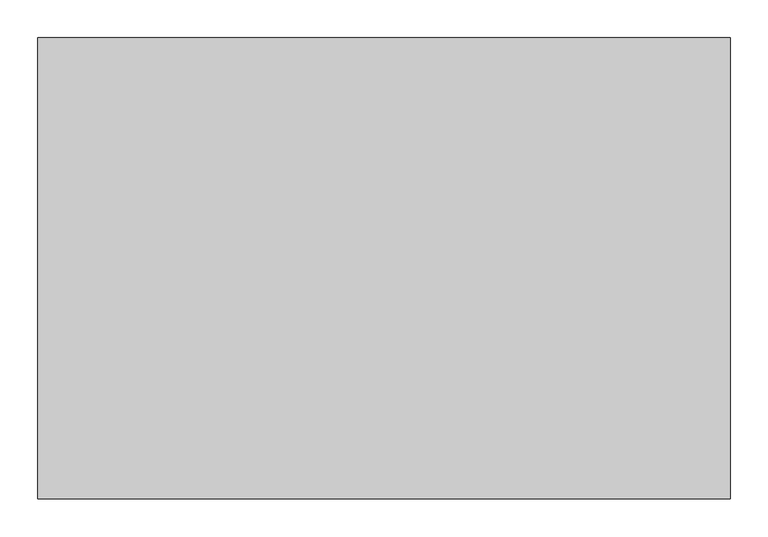
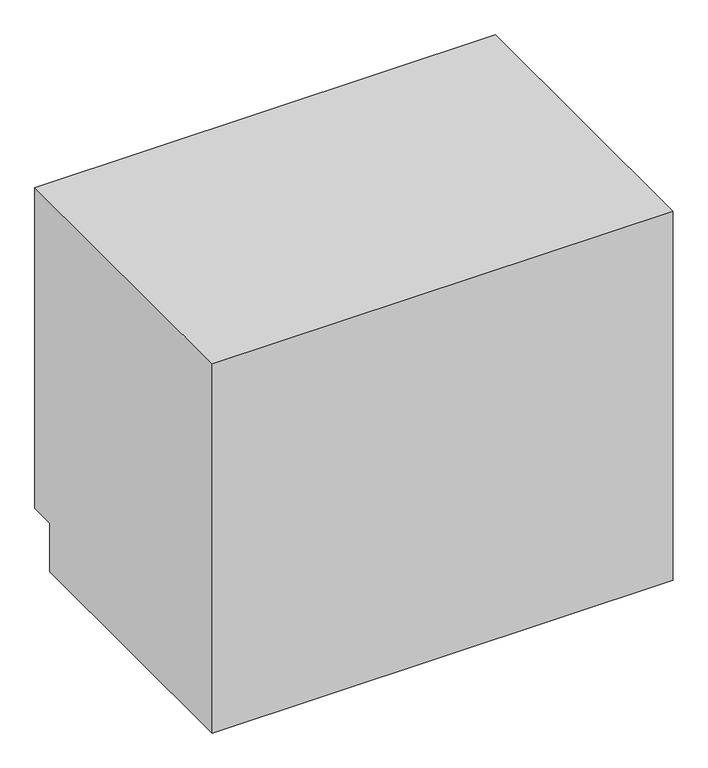
"""IFC4 building model written with IfcOpenShell, lengths in millimetres: furniture geometry, Cabinet, Base Doors and Drawers-NON-COLLECTUS : -."""

from ifc_helpers import new_model, si_unit, frame, origin, place, context, project, spatial, polyline, outline, extrude, source, transform, mapped, element, save


def furniture_34c6b9d5(model_context):
    return source(origin(), model_context, "Body", "SweptSolid", [
        extrude(outline(polyline([(-1384.3, 774.6984506), (-1384.3, 101.6), (-1435.1, 101.6), (-1435.1, 0.0), (-1993.8987808, 0.0), (-1993.8987808, 774.6984506), (-1384.3, 774.6984506)])), frame((114.3, 0.0, 0.0), z_axis=(1.0, 0.0, 0.0), x_axis=(0.0, 1.0, 0.0)), (0.0, 0.0, 1.0), 914.3981712),
    ])


if __name__ == "__main__":
    model = new_model("IFC4")
    model_context = context("Model", 3, world=origin())
    ifc_project = project(units=[si_unit("LENGTHUNIT", "METRE", prefix="MILLI")], contexts=[model_context])
    site = spatial("IfcSite", under=ifc_project)
    building = spatial("IfcBuilding", under=site)
    placement = place(None, origin())
    furniture_shape = furniture_34c6b9d5(model_context)
    element("IfcFurniture", 1, ObjectType="Cabinet, Base Doors and Drawers-NON-COLLECTUS : -", at=placement, inside=building, context=model_context, shape_type="MappedRepresentation", body=[
        mapped(furniture_shape, transform((0.0, 0.0, 0.0), x_axis=(1.0, 0.0, 0.0), y_axis=(0.0, 1.0, 0.0), z_axis=(0.0, 0.0, 1.0))),
    ])
    save(model, "model.ifc")

# Revit data of these elements
# Type "Cabinet, Base Doors and Drawers-NON-COLLECTUS : -"
#   External ID [instance default] = ""
#   Width Reporting [instance default] = 762 mm
#   Width [instance default] = 762 mm
#   Toe Kick Height = 101.6 mm
#   Toe Kick Depth = 50.8 mm
#   Height of Drawers = 152.4 mm
#   Height Reporting [instance default] = 825.5 mm
#   Height [instance default] = 825.5 mm
#   Depth Reporting [instance default] = 609.6 mm
#   Depth [instance default] = 609.6 mm
#   Material = White
#   Default Elevation = 0
# Element 1 (IfcFurniture, "Cabinet, Base Doors and Drawers-NON-COLLECTUS : -")
#   Width Reporting = 914.398 mm
#   Width = 914.398 mm
#   Height Reporting = 774.698 mm
#   Height = 774.698 mm
#   Depth Reporting = 609.599 mm
#   Depth = 609.599 mm
#   Materials on its faces: "White"
# Materials
#   "White": class "Generic", colour RGB 255 255 255, transparency 0, Cost = 0
